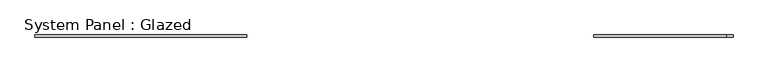
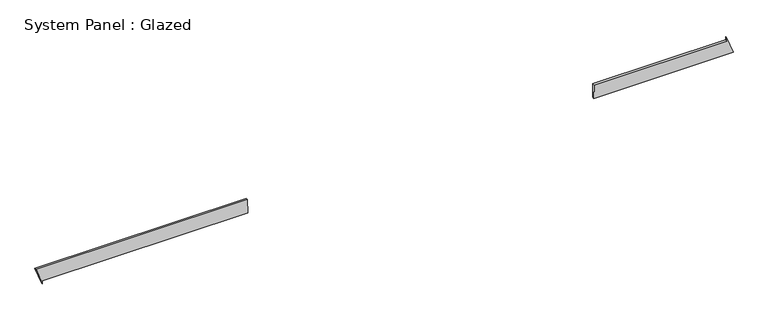
"""IFC4 building model written with IfcOpenShell, lengths in millimetres: plate geometry, System Panel : Glazed."""

from ifc_helpers import new_model, si_unit, frame, origin, place, context, project, spatial, polyline, outline, extrude, source, transform, mapped, element, save


def system_panel_glazed_b9b4df07(model_context):
    return source(origin(), model_context, "Body", "SweptSolid", [
        extrude(outline(polyline([(35.3553391, 2419.4367504), (35.3553391, 4027.6791424), (234.6435672, 3956.3630659), (199.2882281, 3956.3621746), (199.3269257, 2421.2991201), (35.3553391, 2419.4367504)])), frame((0.0, -49.5, 0.0), z_axis=(0.0, 1.0, 0.0), x_axis=(0.0, 0.0, 1.0)), (0.0, 0.0, 1.0), 25.0),
        extrude(outline(polyline([(0.0, -3956.8326568), (35.3553391, -3956.8326568), (35.3553391, -1584.573302), (199.4279412, -1585.80098), (199.4894988, -4027.6791424), (0.0, -3956.8326568)])), frame((0.0, -49.5, 0.0), z_axis=(0.0, 1.0, 0.0), x_axis=(0.0, 0.0, 1.0)), (0.0, 0.0, 1.0), 25.0),
    ])


if __name__ == "__main__":
    model = new_model("IFC4")
    model_context = context("Model", 3, world=origin())
    ifc_project = project(units=[si_unit("LENGTHUNIT", "METRE", prefix="MILLI")], contexts=[model_context])
    site = spatial("IfcSite", under=ifc_project)
    building = spatial("IfcBuilding", under=site)
    placement = place(None, origin())
    system_panel_glazed_shape = system_panel_glazed_b9b4df07(model_context)
    element("IfcPlate", 1, ObjectType="System Panel : Glazed", at=placement, inside=building, context=model_context, shape_type="MappedRepresentation", body=[
        mapped(system_panel_glazed_shape, transform((0.0, 0.0, 0.0), x_axis=(1.0, 0.0, 0.0), y_axis=(0.0, 1.0, 0.0), z_axis=(0.0, 0.0, 1.0))),
    ])
    save(model, "model.ifc")

# Revit data of these elements
# Element 1 (IfcPlate, "System Panel : Glazed")
#   Materials on its faces: "Glass"
# Materials
#   "Glass": class "Glass", colour RGB 218 227 224, transparency 0.85, Description = "Soda Lime Glass", Cost = 0
